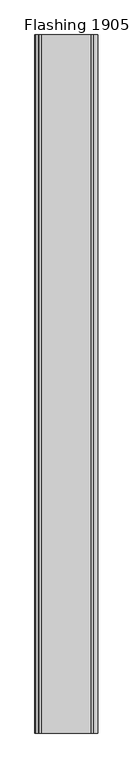
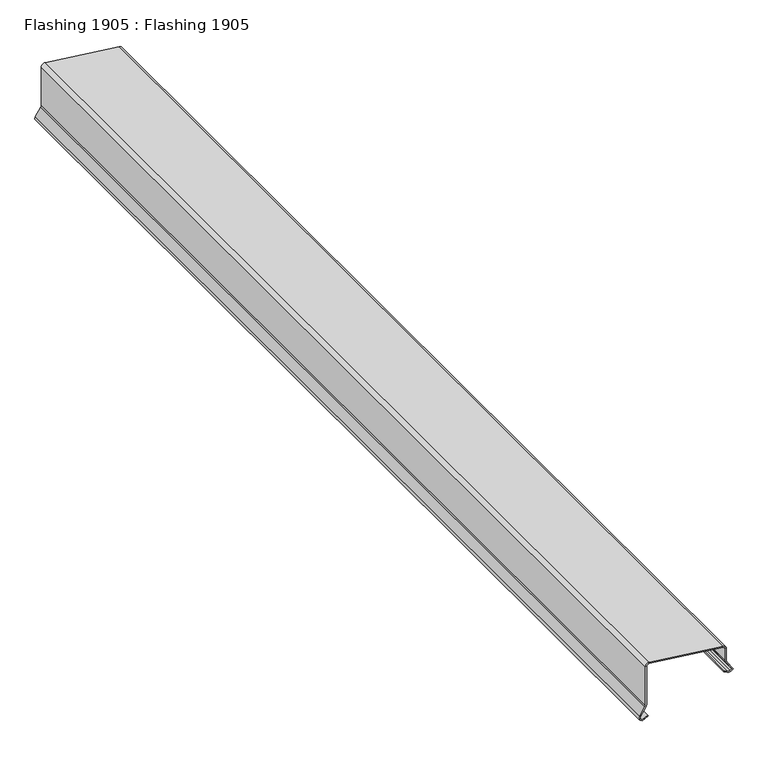
"""IFC4 building model written with IfcOpenShell, lengths in millimetres: proxy geometry, Flashing 1905 : Flashing 1905."""

from ifc_helpers import new_model, si_unit, point, frame, frame_2d, origin, place, context, project, spatial, polyline, circle_curve, trimmed, segment, composite_curve, outline, extrude, source, transform, mapped, element, save


def flashing_1905_flashing_1905_d6e76b17(model_context):
    return source(origin(), model_context, "Body", "SweptSolid", [
        extrude(outline(composite_curve([segment(trimmed(circle_curve(frame_2d((40133.2517994, -9767.0036771)), 6.35), [point((40127.5360053, -9769.7699376))], [point((40127.867313, -9763.6376994))], False, "CARTESIAN"), True, "CONTINUOUS"), segment(polyline([(40127.867313, -9763.6376994), (40130.8867187, -9758.8076172), (40149.4789842, -9770.8014653)]), True, "CONTINUOUS"), segment(trimmed(circle_curve(frame_2d((40152.9212544, -9765.4654297)), 6.35), [point((40149.4789842, -9770.8014653))], [point((40152.9212544, -9771.8154297))], True, "CARTESIAN"), True, "CONTINUOUS"), segment(polyline([(40152.9212544, -9771.8154297), (40176.1640916, -9771.8154297)]), True, "CONTINUOUS"), segment(trimmed(circle_curve(frame_2d((40176.1640916, -9778.1654297)), 6.35), [point((40176.1640916, -9771.8154297))], [point((40182.4677067, -9777.3993118))], False, "CARTESIAN"), True, "CONTINUOUS"), segment(polyline([(40182.4677067, -9777.3993118), (40199.6976336, -9919.1670852)]), True, "CONTINUOUS"), segment(trimmed(circle_curve(frame_2d((40193.3940184, -9919.9332031)), 6.35), [point((40199.6976336, -9919.1670852))], [point((40193.3940184, -9926.2832031))], False, "CARTESIAN"), True, "CONTINUOUS"), segment(polyline([(40193.3940184, -9926.2832031), (40116.1659228, -9926.2832031)]), True, "CONTINUOUS"), segment(trimmed(circle_curve(frame_2d((40116.1659228, -9932.6332031)), 6.35), [point((40116.1659228, -9926.2832031))], [point((40112.7319037, -9927.2918538))], True, "CARTESIAN"), True, "CONTINUOUS"), segment(polyline([(40112.7319037, -9927.2918538), (40096.8914441, -9937.4758802)]), True, "CONTINUOUS"), segment(trimmed(circle_curve(frame_2d((40093.4574249, -9932.1345309)), 6.35), [point((40096.8914441, -9937.4758802))], [point((40088.1090015, -9935.5575219))], False, "CARTESIAN"), True, "CONTINUOUS"), segment(polyline([(40088.1090015, -9935.5575219), (40086.3359375, -9932.7871094), (40092.1875, -9921.0800781), (40093.9764738, -9921.9742665), (40088.63264, -9932.6655014), (40089.7935443, -9934.4794145)]), True, "CONTINUOUS"), segment(trimmed(circle_curve(frame_2d((40093.4574249, -9932.1345309)), 4.35), [point((40089.7935443, -9934.4794145))], [point((40095.8098632, -9935.7935655))], True, "CARTESIAN"), True, "CONTINUOUS"), segment(polyline([(40095.8098632, -9935.7935655), (40111.6503228, -9925.6095391)]), True, "CONTINUOUS"), segment(trimmed(circle_curve(frame_2d((40116.1659228, -9932.6332031)), 8.35), [point((40111.6503228, -9925.6095391))], [point((40116.1659228, -9924.2832031))], False, "CARTESIAN"), True, "CONTINUOUS"), segment(polyline([(40116.1659228, -9924.2832031), (40193.3940184, -9924.2832031)]), True, "CONTINUOUS"), segment(trimmed(circle_curve(frame_2d((40193.3940184, -9919.9332031)), 4.35), [point((40193.3940184, -9924.2832031))], [point((40197.712243, -9919.4083822))], True, "CARTESIAN"), True, "CONTINUOUS"), segment(polyline([(40197.712243, -9919.4083822), (40180.4823161, -9777.6406088)]), True, "CONTINUOUS"), segment(trimmed(circle_curve(frame_2d((40176.1640916, -9778.1654297)), 4.35), [point((40180.4823161, -9777.6406088))], [point((40176.1640916, -9773.8154297))], True, "CARTESIAN"), True, "CONTINUOUS"), segment(polyline([(40176.1640916, -9773.8154297), (40152.9212544, -9773.8154297)]), True, "CONTINUOUS"), segment(trimmed(circle_curve(frame_2d((40152.9212544, -9765.4654297)), 8.35), [point((40152.9212544, -9773.8154297))], [point((40148.3948046, -9772.4821064))], False, "CARTESIAN"), True, "CONTINUOUS"), segment(polyline([(40148.3948046, -9772.4821064), (40131.5072723, -9761.5879796), (40129.5632143, -9764.6978498)]), True, "CONTINUOUS"), segment(trimmed(circle_curve(frame_2d((40133.2517994, -9767.0036771)), 4.35), [point((40129.5632143, -9764.6978498))], [point((40129.3362554, -9768.8986745))], True, "CARTESIAN"), True, "CONTINUOUS"), segment(polyline([(40129.3362554, -9768.8986745), (40132.6869689, -9775.8220962), (40130.8867187, -9776.6933594), (40127.5360053, -9769.7699376)]), True, "CONTINUOUS")], self_intersect=False)), frame((0.0, 7982.1531721, 0.0), z_axis=(0.0, 1.0, 0.0), x_axis=(0.0, 0.0, 1.0)), (0.0, 0.0, 1.0), 2000.0),
    ])


if __name__ == "__main__":
    model = new_model("IFC4")
    model_context = context("Model", 3, world=origin())
    ifc_project = project(units=[si_unit("LENGTHUNIT", "METRE", prefix="MILLI")], contexts=[model_context])
    site = spatial("IfcSite", under=ifc_project)
    building = spatial("IfcBuilding", under=site)
    placement = place(None, origin())
    flashing_1905_flashing_1905_shape = flashing_1905_flashing_1905_d6e76b17(model_context)
    element("IfcBuildingElementProxy", 1, Name="Flashing 1905 : Flashing 1905", ObjectType="Flashing 1905 : Flashing 1905", at=placement, inside=building, context=model_context, shape_type="MappedRepresentation", body=[
        mapped(flashing_1905_flashing_1905_shape, transform((0.0, 0.0, 0.0), x_axis=(1.0, 0.0, 0.0), y_axis=(0.0, 1.0, 0.0), z_axis=(0.0, 0.0, 1.0))),
    ])
    save(model, "model.ifc")

# Revit data of these elements
# Type "Flashing 1905 : Flashing 1905"
#   NameOverride = "Flashing"
# Element 1 (IfcBuildingElementProxy, "Flashing 1905 : Flashing 1905")
#   Materials on its faces: "METAL COPING"
# Materials
#   "METAL COPING": class "Unassigned", colour RGB 128 128 128, transparency 0
